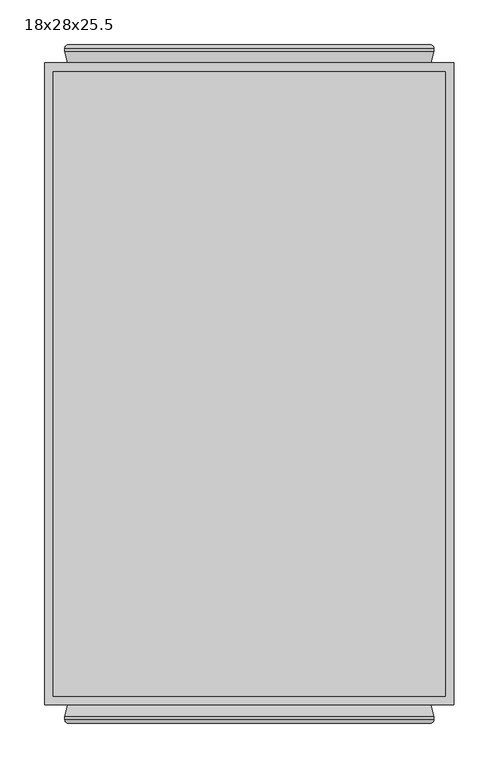
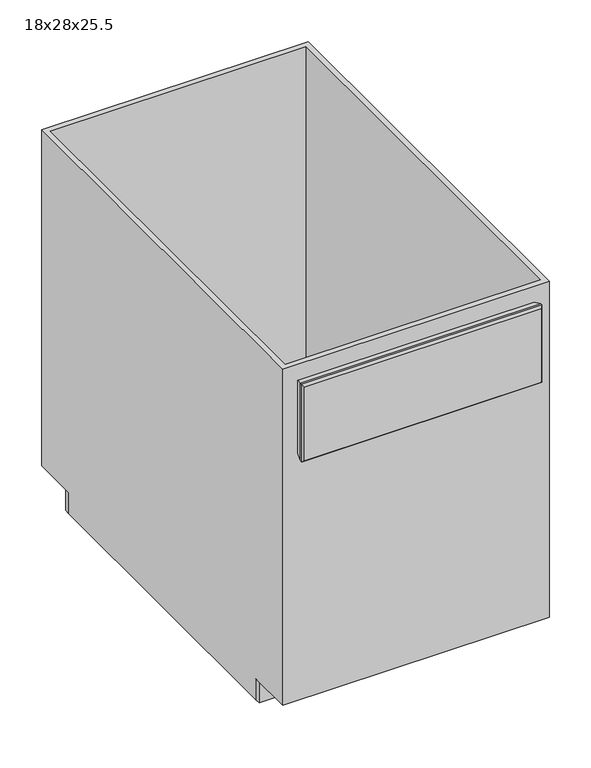
"""IFC4 building model written with IfcOpenShell, lengths in millimetres: furniture geometry, Cabinet-Base-Merillat-Peninsula_Single_Door-Marlin : 18x28x25.5."""

from ifc_helpers import new_model, si_unit, frame, origin, origin_with_axes, place, context, project, spatial, polyline, circle_curve, ellipse_curve, outline, extrude, faceted_brep, source, transform, mapped, element, save
from ifc_brep_helpers import plane_surface, cylinder_surface, advanced_brep


def furniture_18x28x25_5_8da4ed4e(model_context):
    return source(origin(), model_context, "Body", "SolidModel", [
        advanced_brep(
        [(225.1127049, 52.3621, 63.5), (222.0162124, 56.8325, 66.5964925), (222.0162124, 56.8325, 454.1035075), (225.1127049, 52.3621, 457.2), (225.1127049, 49.5935, 457.2), (225.1127049, 49.5935, 63.5), (221.6075049, 36.5125, 453.6948), (221.6075049, 36.5125, 67.0052), (176.9115422, 36.5125, 111.7011628), (176.9115422, 36.5125, 408.9988372), (176.5414105, 37.30625, 408.6287055), (174.4602514, 41.76931, 406.5475465), (174.4602514, 41.76931, 114.1524535), (176.5414105, 37.30625, 112.0712945), (175.8600209, 44.0094093, 407.947316), (175.8600209, 44.0094093, 112.752684), (190.1877049, 44.2595, 422.275), (190.1877049, 44.2595, 98.425), (190.1877049, 49.0855, 422.275), (190.1877049, 49.0855, 98.425), (175.8600209, 49.3355907, 407.947316), (175.8600209, 49.3355907, 112.752684), (174.4602514, 51.57569, 406.5475465), (174.4602514, 51.57569, 114.1524535), (176.5414105, 56.03875, 408.6287055), (176.9086747, 56.8263508, 408.9959698), (176.9115422, 56.8325, 111.7011628), (176.5414105, 56.03875, 112.0712945), (176.9086747, 56.8325, 454.1035075), (176.9086747, 52.3621, 457.2), (-184.5408026, 56.8325, 454.1035075), (-187.6372951, 52.3621, 457.2), (-139.4730764, 52.3621, 457.2), (-139.4730764, 56.8325, 454.1035075), (175.3211747, 52.3621, 457.2), (175.3211747, 56.8325, 454.1035075), (-137.8855764, 56.8325, 454.1035075), (-137.8855764, 52.3621, 457.2), (176.9086747, 49.5935, 457.2), (-187.6372951, 49.5935, 457.2), (-139.4730764, 49.5935, 457.2), (175.3211747, 49.5935, 457.2), (-137.8855764, 49.5935, 457.2), (176.9086747, 36.5125, 453.6948), (-184.1320951, 36.5125, 453.6948), (-139.4730764, 36.5125, 453.6948), (175.3211747, 36.5125, 453.6948), (-137.8855764, 36.5125, 453.6948), (-136.9848416, 41.76931, 406.5475465), (175.3211747, 37.30625, 408.6287055), (175.3211747, 36.5125, 408.9988372), (-137.8855764, 36.5125, 408.9988372), (-137.8855764, 37.30625, 408.6287055), (-139.0660006, 37.30625, 408.6287055), (-138.384611, 44.0094093, 407.947316), (-152.7122951, 44.2595, 422.275), (-152.7122951, 49.0855, 422.275), (-138.384611, 49.3355907, 407.947316), (-136.9848416, 51.57569, 406.5475465), (-139.0660006, 56.03875, 408.6287055), (-137.8855764, 56.03875, 408.6287055), (-137.8855764, 56.8325, 408.9988372), (175.3211747, 56.8325, 408.9988372), (175.3211747, 56.03875, 408.6287055), (-184.5408026, 56.8325, 66.5964925), (-187.6372951, 52.3621, 63.5), (-187.6372951, 49.5935, 63.5), (-184.1320951, 36.5125, 67.0052), (-139.4361323, 36.5125, 408.9988372), (-139.4361323, 36.5125, 111.7011628), (-139.0660006, 37.30625, 112.0712945), (-136.9848416, 41.76931, 114.1524535), (-138.384611, 44.0094093, 112.752684), (-152.7122951, 44.2595, 98.425), (-152.7122951, 49.0855, 98.425), (-138.384611, 49.3355907, 112.752684), (-136.9848416, 51.57569, 114.1524535), (-139.0660006, 56.03875, 112.0712945), (-139.4361323, 56.8325, 111.7011628), (-139.4361323, 56.8325, 408.9988372), (-139.4730764, 56.8325, 66.5964925), (-139.4730764, 52.3621, 63.5), (176.9086747, 52.3621, 63.5), (176.9086747, 56.8325, 66.5964925), (-137.8855764, 52.3621, 63.5), (-137.8855764, 56.8325, 66.5964925), (175.3211747, 56.8325, 66.5964925), (175.3211747, 52.3621, 63.5), (-139.4730764, 49.5935, 63.5), (176.9086747, 49.5935, 63.5), (-137.8855764, 49.5935, 63.5), (175.3211747, 49.5935, 63.5), (-139.4730764, 36.5125, 67.0052), (176.9086747, 36.5125, 67.0052), (-137.8855764, 36.5125, 67.0052), (175.3211747, 36.5125, 67.0052), (-137.8855764, 36.5125, 111.7011628), (175.3211747, 36.5125, 111.7011628), (-137.8855764, 37.30625, 112.0712945), (175.3211747, 37.30625, 112.0712945), (175.3211747, 56.03875, 112.0712945), (175.3211747, 56.8325, 111.7011628), (-137.8855764, 56.8325, 111.7011628), (-137.8855764, 56.03875, 112.0712945), (-137.8855764, 37.30625, 67.6142588), (-137.8855764, 49.6980037, 64.29375), (-137.8855764, 52.3621, 64.29375), (-137.8855764, 56.03875, 66.7473948), (-139.4730764, 56.03875, 112.0712945), (-139.4730764, 56.03875, 66.7473948), (-139.4730764, 52.3621, 64.29375), (-139.4730764, 49.6980037, 64.29375), (-139.4730764, 37.30625, 67.6142588), (-139.4730764, 37.30625, 112.0712945), (176.9086747, 37.30625, 112.0712945), (176.9086747, 37.30625, 67.6142588), (176.9086747, 49.6980037, 64.29375), (176.9086747, 52.3621, 64.29375), (176.9086747, 56.03875, 66.7473948), (176.9086747, 56.03875, 112.0712945), (175.3211747, 56.03875, 66.7473948), (175.3211747, 52.3621, 64.29375), (175.3211747, 49.6980037, 64.29375), (175.3211747, 37.30625, 67.6142588), (176.9086747, 56.03875, 408.6287055), (176.9086747, 56.03875, 453.9526052), (176.9086747, 52.3621, 456.40625), (176.9086747, 49.6980037, 456.40625), (176.9086747, 37.30625, 453.0857412), (176.9086747, 37.30625, 408.6287055), (175.3211747, 37.30625, 453.0857412), (175.3211747, 49.6980037, 456.40625), (175.3211747, 52.3621, 456.40625), (175.3211747, 56.03875, 453.9526052), (-137.8855764, 56.03875, 453.9526052), (-137.8855764, 52.3621, 456.40625), (-137.8855764, 49.6980037, 456.40625), (-137.8855764, 37.30625, 453.0857412), (-139.4730764, 56.03875, 408.6287055), (-139.4730764, 37.30625, 408.6287055), (-139.4730764, 37.30625, 453.0857412), (-139.4730764, 49.6980037, 456.40625), (-139.4730764, 52.3621, 456.40625), (-139.4730764, 56.03875, 453.9526052)],
        [
            (0, 1, ellipse_curve(frame((220.3375049, 52.3621, 68.2752), z_axis=(0.7071067811865498, 0.0, 0.7071067811865451), x_axis=(0.7071067811865451, 0.0, -0.70710678118655)), 6.7531526, 4.7752)),
            (1, 2),
            (2, 3, ellipse_curve(frame((220.3375049, 52.3621, 452.4248), z_axis=(0.7071067811865451, 0.0, -0.7071067811865498), x_axis=(-0.7071067811865497, 0.0, -0.7071067811865452)), 6.7531526, 4.7752)),
            (3, 0),
            (3, 4),
            (4, 5),
            (5, 0),
            (4, 6),
            (6, 7),
            (7, 5),
            (8, 9),
            (9, 10),
            (10, 11),
            (11, 12),
            (12, 13),
            (13, 8),
            (11, 14, ellipse_curve(frame((175.8875049, 42.4348492, 407.9748), z_axis=(0.7071067811865451, 0.0, -0.7071067811865498), x_axis=(-0.7071067811865497, 0.0, -0.7071067811865452)), 2.2271035, 1.5748)),
            (14, 15),
            (15, 12, ellipse_curve(frame((175.8875049, 42.4348492, 112.7252), z_axis=(0.7071067811865498, 0.0, 0.7071067811865451), x_axis=(0.7071067811865451, 0.0, -0.70710678118655)), 2.2271035, 1.5748)),
            (14, 16),
            (16, 17),
            (17, 15),
            (16, 18),
            (18, 19),
            (19, 17),
            (18, 20),
            (20, 21),
            (21, 19),
            (20, 22, ellipse_curve(frame((175.8875049, 50.9101508, 407.9748), z_axis=(0.7071067811865451, 0.0, -0.7071067811865498), x_axis=(-0.7071067811865497, 0.0, -0.7071067811865452)), 2.2271035, 1.5748)),
            (22, 23),
            (23, 21, ellipse_curve(frame((175.8875049, 50.9101508, 112.7252), z_axis=(0.7071067811865498, 0.0, 0.7071067811865451), x_axis=(0.7071067811865451, 0.0, -0.70710678118655)), 2.2271035, 1.5748)),
            (22, 24),
            (24, 25),
            (25, 26),
            (26, 27),
            (27, 23),
            (2, 28),
            (28, 29, circle_curve(frame((176.9086747, 52.3621, 452.4248), z_axis=(1.0, 0.0, 0.0), x_axis=(0.0, -1.0, 0.0)), 4.7752)),
            (29, 3),
            (30, 31, ellipse_curve(frame((-182.8620951, 52.3621, 452.4248), z_axis=(0.7071067811865498, 0.0, 0.7071067811865451), x_axis=(0.7071067811865452, 0.0, -0.7071067811865497)), 6.7531526, 4.7752)),
            (31, 32),
            (32, 33, circle_curve(frame((-139.4730764, 52.3621, 452.4248), z_axis=(-1.0, 0.0, 0.0), x_axis=(0.0, -1.0, 0.0)), 4.7752)),
            (33, 30),
            (34, 35, circle_curve(frame((175.3211747, 52.3621, 452.4248), z_axis=(-1.0, 0.0, 0.0), x_axis=(0.0, -1.0, 0.0)), 4.7752)),
            (35, 36),
            (36, 37, circle_curve(frame((-137.8855764, 52.3621, 452.4248), z_axis=(1.0, 0.0, 0.0), x_axis=(0.0, -1.0, 0.0)), 4.7752)),
            (37, 34),
            (29, 38),
            (38, 4),
            (31, 39),
            (39, 40),
            (40, 32),
            (41, 34),
            (37, 42),
            (42, 41),
            (38, 43),
            (43, 6),
            (39, 44),
            (44, 45),
            (45, 40),
            (46, 41),
            (42, 47),
            (47, 46),
            (48, 11),
            (10, 49),
            (49, 50),
            (50, 51),
            (51, 52),
            (52, 53),
            (53, 48),
            (48, 54, ellipse_curve(frame((-138.4120951, 42.4348492, 407.9748), z_axis=(0.7071067811865498, 0.0, 0.7071067811865451), x_axis=(0.7071067811865452, 0.0, -0.7071067811865497)), 2.2271035, 1.5748)),
            (54, 14),
            (54, 55),
            (55, 16),
            (55, 56),
            (56, 18),
            (56, 57),
            (57, 20),
            (57, 58, ellipse_curve(frame((-138.4120951, 50.9101508, 407.9748), z_axis=(0.7071067811865498, 0.0, 0.7071067811865451), x_axis=(0.7071067811865452, 0.0, -0.7071067811865497)), 2.2271035, 1.5748)),
            (58, 22),
            (58, 59),
            (59, 60),
            (60, 61),
            (61, 62),
            (62, 63),
            (63, 24),
            (30, 64),
            (64, 65, ellipse_curve(frame((-182.8620951, 52.3621, 68.2752), z_axis=(-0.7071067811865451, 0.0, 0.7071067811865498), x_axis=(0.7071067811865497, 0.0, 0.7071067811865452)), 6.7531526, 4.7752)),
            (65, 31),
            (65, 66),
            (66, 39),
            (66, 67),
            (67, 44),
            (68, 69),
            (69, 70),
            (70, 71),
            (71, 48),
            (53, 68),
            (71, 72, ellipse_curve(frame((-138.4120951, 42.4348492, 112.7252), z_axis=(-0.7071067811865451, 0.0, 0.7071067811865498), x_axis=(0.7071067811865497, 0.0, 0.7071067811865452)), 2.2271035, 1.5748)),
            (72, 54),
            (72, 73),
            (73, 55),
            (73, 74),
            (74, 56),
            (74, 75),
            (75, 57),
            (75, 76, ellipse_curve(frame((-138.4120951, 50.9101508, 112.7252), z_axis=(-0.7071067811865451, 0.0, 0.7071067811865498), x_axis=(0.7071067811865497, 0.0, 0.7071067811865452)), 2.2271035, 1.5748)),
            (76, 58),
            (76, 77),
            (77, 78),
            (78, 79),
            (79, 59),
            (64, 80),
            (80, 81, circle_curve(frame((-139.4730764, 52.3621, 68.2752), z_axis=(-1.0, 0.0, 0.0), x_axis=(0.0, -1.0, 0.0)), 4.7752)),
            (81, 65),
            (0, 82),
            (82, 83, circle_curve(frame((176.9086747, 52.3621, 68.2752), z_axis=(1.0, 0.0, 0.0), x_axis=(0.0, -1.0, 0.0)), 4.7752)),
            (83, 1),
            (84, 85, circle_curve(frame((-137.8855764, 52.3621, 68.2752), z_axis=(1.0, 0.0, 0.0), x_axis=(0.0, -1.0, 0.0)), 4.7752)),
            (85, 86),
            (86, 87, circle_curve(frame((175.3211747, 52.3621, 68.2752), z_axis=(-1.0, 0.0, 0.0), x_axis=(0.0, -1.0, 0.0)), 4.7752)),
            (87, 84),
            (81, 88),
            (88, 66),
            (5, 89),
            (89, 82),
            (90, 84),
            (87, 91),
            (91, 90),
            (88, 92),
            (92, 67),
            (7, 93),
            (93, 89),
            (94, 90),
            (91, 95),
            (95, 94),
            (43, 9),
            (8, 93),
            (92, 69),
            (68, 45),
            (96, 94),
            (95, 97),
            (97, 96),
            (50, 46),
            (47, 51),
            (12, 71),
            (70, 98),
            (98, 96),
            (97, 99),
            (99, 13),
            (15, 72),
            (17, 73),
            (19, 74),
            (21, 75),
            (23, 76),
            (27, 100),
            (100, 101),
            (101, 102),
            (102, 103),
            (103, 77),
            (83, 26),
            (25, 28),
            (33, 79),
            (78, 80),
            (85, 102),
            (101, 86),
            (35, 62),
            (61, 36),
            (98, 104),
            (104, 105),
            (105, 106),
            (106, 107, circle_curve(frame((-137.8855764, 52.3621, 68.2752), z_axis=(1.0, 0.0, 0.0), x_axis=(0.0, 0.0, -1.0)), 3.98145)),
            (107, 103),
            (78, 108),
            (108, 109),
            (109, 110, circle_curve(frame((-139.4730764, 52.3621, 68.2752), z_axis=(-1.0, 0.0, 0.0), x_axis=(0.0, 0.0, -1.0)), 3.98145)),
            (110, 111),
            (111, 112),
            (112, 113),
            (113, 69),
            (77, 108),
            (107, 109),
            (106, 110),
            (105, 111),
            (104, 112),
            (70, 113),
            (8, 114),
            (114, 115),
            (115, 116),
            (116, 117),
            (117, 118, circle_curve(frame((176.9086747, 52.3621, 68.2752), z_axis=(1.0, 0.0, 0.0), x_axis=(0.0, 0.0, -1.0)), 3.98145)),
            (118, 119),
            (119, 26),
            (100, 120),
            (120, 121, circle_curve(frame((175.3211747, 52.3621, 68.2752), z_axis=(-1.0, 0.0, 0.0), x_axis=(0.0, 0.0, -1.0)), 3.98145)),
            (121, 122),
            (122, 123),
            (123, 99),
            (119, 27),
            (118, 120),
            (117, 121),
            (116, 122),
            (115, 123),
            (114, 13),
            (25, 124),
            (124, 125),
            (125, 126, circle_curve(frame((176.9086747, 52.3621, 452.4248), z_axis=(1.0, 0.0, 0.0), x_axis=(0.0, 0.0, -1.0)), 3.98145)),
            (126, 127),
            (127, 128),
            (128, 129),
            (129, 9),
            (49, 130),
            (130, 131),
            (131, 132),
            (132, 133, circle_curve(frame((175.3211747, 52.3621, 452.4248), z_axis=(-1.0, 0.0, 0.0), x_axis=(0.0, 0.0, -1.0)), 3.98145)),
            (133, 63),
            (129, 10),
            (128, 130),
            (127, 131),
            (126, 132),
            (125, 133),
            (124, 24),
            (60, 134),
            (134, 135, circle_curve(frame((-137.8855764, 52.3621, 452.4248), z_axis=(1.0, 0.0, 0.0), x_axis=(0.0, 0.0, -1.0)), 3.98145)),
            (135, 136),
            (136, 137),
            (137, 52),
            (138, 79),
            (68, 139),
            (139, 140),
            (140, 141),
            (141, 142),
            (142, 143, circle_curve(frame((-139.4730764, 52.3621, 452.4248), z_axis=(-1.0, 0.0, 0.0), x_axis=(0.0, 0.0, -1.0)), 3.98145)),
            (143, 138),
            (138, 59),
            (53, 139),
            (137, 140),
            (136, 141),
            (135, 142),
            (134, 143),
        ],
        [
            cylinder_surface(frame((220.3375049, 52.3621, 63.5), z_axis=(0.0, 0.0, -1.0), x_axis=(0.0, -1.0, 0.0)), 4.7752),
            plane_surface(frame((225.1127049, 52.3621, 63.5), z_axis=(1.0, 0.0, 0.0), x_axis=(0.0, 0.0, 1.0))),
            plane_surface(frame((225.1127049, 49.5935, 63.5), z_axis=(0.9659229350723619, -0.25882983502910506, 0.0), x_axis=(0.0, 0.0, 1.0))),
            plane_surface(frame((176.9115422, 36.5125, 111.7011628), z_axis=(-0.9063077870366099, -0.4226182617407856, 0.0), x_axis=(0.0, 0.0, 1.0))),
            cylinder_surface(frame((175.8875049, 42.4348492, 63.5), z_axis=(0.0, 0.0, -1.0000000000000002), x_axis=(-0.01745240643729364, 0.9998476951563912, 0.0)), 1.5748),
            plane_surface(frame((175.8600209, 44.0094093, 112.752684), z_axis=(-0.017452406437322144, 0.9998476951563906, 0.0), x_axis=(0.0, 0.0, 1.0))),
            plane_surface(frame((190.1877049, 44.2595, 98.425), z_axis=(-1.0, 0.0, 0.0), x_axis=(0.0, 0.0, 1.0))),
            plane_surface(frame((190.1877049, 49.0855, 98.425), z_axis=(-0.01745240643727848, -0.9998476951563914, 0.0), x_axis=(0.0, 0.0, 1.0))),
            cylinder_surface(frame((175.8875049, 50.9101508, 63.5), z_axis=(0.0, 0.0, -1.0000000000000002), x_axis=(-0.9063077870367326, 0.42261826174052236, 0.0)), 1.5748),
            plane_surface(frame((174.4602514, 51.57569, 114.1524535), z_axis=(-0.9063077870366333, 0.4226182617407352, 0.0), x_axis=(0.0, 0.0, 1.0))),
            cylinder_surface(frame((225.1127049, 52.3621, 452.4248), z_axis=(1.0, 0.0, 0.0), x_axis=(0.0, -1.0, 0.0)), 4.7752),
            plane_surface(frame((225.1127049, 52.3621, 457.2), z_axis=(0.0, 0.0, 1.0), x_axis=(-1.0, 0.0, 0.0))),
            plane_surface(frame((225.1127049, 49.5935, 457.2), z_axis=(0.0, -0.25882983502910506, 0.9659229350723619), x_axis=(-1.0, 0.0, 0.0))),
            plane_surface(frame((176.9115422, 36.5125, 408.9988372), z_axis=(0.0, -0.4226182617407856, -0.9063077870366099), x_axis=(-1.0, 0.0, 0.0))),
            cylinder_surface(frame((225.1127049, 42.4348492, 407.9748), z_axis=(1.0000000000000002, 0.0, 0.0), x_axis=(0.0, 0.9998476951563912, -0.01745240643729364)), 1.5748),
            plane_surface(frame((175.8600209, 44.0094093, 407.947316), z_axis=(0.0, 0.9998476951563906, -0.017452406437322144), x_axis=(-1.0, 0.0, 0.0))),
            plane_surface(frame((190.1877049, 44.2595, 422.275), z_axis=(0.0, 0.0, -1.0), x_axis=(-1.0, 0.0, 0.0))),
            plane_surface(frame((190.1877049, 49.0855, 422.275), z_axis=(0.0, -0.9998476951563914, -0.01745240643727848), x_axis=(-1.0, 0.0, 0.0))),
            cylinder_surface(frame((225.1127049, 50.9101508, 407.9748), z_axis=(1.0000000000000002, 0.0, 0.0), x_axis=(0.0, 0.42261826174052236, -0.9063077870367326)), 1.5748),
            plane_surface(frame((174.4602514, 51.57569, 406.5475465), z_axis=(0.0, 0.4226182617407352, -0.9063077870366333), x_axis=(-1.0, 0.0, 0.0))),
            cylinder_surface(frame((-182.8620951, 52.3621, 457.2), z_axis=(0.0, 0.0, 1.0), x_axis=(0.0, -1.0, 0.0)), 4.7752),
            plane_surface(frame((-187.6372951, 52.3621, 457.2), z_axis=(-1.0, 0.0, 0.0), x_axis=(0.0, 0.0, -1.0))),
            plane_surface(frame((-187.6372951, 49.5935, 457.2), z_axis=(-0.9659229350723619, -0.25882983502910506, 0.0), x_axis=(0.0, 0.0, -1.0))),
            plane_surface(frame((-139.4361323, 36.5125, 408.9988372), z_axis=(0.9063077870366099, -0.4226182617407856, 0.0), x_axis=(0.0, 0.0, -1.0))),
            cylinder_surface(frame((-138.4120951, 42.4348492, 457.2), z_axis=(0.0, 0.0, 1.0000000000000002), x_axis=(0.01745240643729364, 0.9998476951563912, 0.0)), 1.5748),
            plane_surface(frame((-138.384611, 44.0094093, 407.947316), z_axis=(0.017452406437322144, 0.9998476951563906, 0.0), x_axis=(0.0, 0.0, -1.0))),
            plane_surface(frame((-152.7122951, 44.2595, 422.275), z_axis=(1.0, 0.0, 0.0), x_axis=(0.0, 0.0, -1.0))),
            plane_surface(frame((-152.7122951, 49.0855, 422.275), z_axis=(0.01745240643727848, -0.9998476951563914, 0.0), x_axis=(0.0, 0.0, -1.0))),
            cylinder_surface(frame((-138.4120951, 50.9101508, 457.2), z_axis=(0.0, 0.0, 1.0000000000000002), x_axis=(0.9063077870367326, 0.42261826174052236, 0.0)), 1.5748),
            plane_surface(frame((-136.9848416, 51.57569, 406.5475465), z_axis=(0.9063077870366333, 0.4226182617407352, 0.0), x_axis=(0.0, 0.0, -1.0))),
            cylinder_surface(frame((-187.6372951, 52.3621, 68.2752), z_axis=(-1.0, 0.0, 0.0), x_axis=(0.0, -1.0, 0.0)), 4.7752),
            plane_surface(frame((-187.6372951, 52.3621, 63.5), z_axis=(0.0, 0.0, -1.0), x_axis=(1.0, 0.0, 0.0))),
            plane_surface(frame((-187.6372951, 49.5935, 63.5), z_axis=(0.0, -0.25882983502910506, -0.9659229350723619), x_axis=(1.0, 0.0, 0.0))),
            plane_surface(frame((-184.1320951, 36.5125, 67.0052), z_axis=(0.0, -1.0, 0.0), x_axis=(1.0, 0.0, 0.0))),
            plane_surface(frame((-139.4361323, 36.5125, 111.7011628), z_axis=(0.0, -0.4226182617407856, 0.9063077870366099), x_axis=(1.0, 0.0, 0.0))),
            cylinder_surface(frame((-187.6372951, 42.4348492, 112.7252), z_axis=(-1.0000000000000002, 0.0, 0.0), x_axis=(0.0, 0.9998476951563912, 0.01745240643729364)), 1.5748),
            plane_surface(frame((-138.384611, 44.0094093, 112.752684), z_axis=(0.0, 0.9998476951563906, 0.017452406437322144), x_axis=(1.0, 0.0, 0.0))),
            plane_surface(frame((-152.7122951, 44.2595, 98.425), z_axis=(0.0, 0.0, 1.0), x_axis=(1.0, 0.0, 0.0))),
            plane_surface(frame((-152.7122951, 49.0855, 98.425), z_axis=(0.0, -0.9998476951563914, 0.01745240643727848), x_axis=(1.0, 0.0, 0.0))),
            cylinder_surface(frame((-187.6372951, 50.9101508, 112.7252), z_axis=(-1.0000000000000002, 0.0, 0.0), x_axis=(0.0, 0.42261826174052236, 0.9063077870367326)), 1.5748),
            plane_surface(frame((-136.9848416, 51.57569, 114.1524535), z_axis=(0.0, 0.4226182617407352, 0.9063077870366333), x_axis=(1.0, 0.0, 0.0))),
            plane_surface(frame((-139.4361323, 56.8325, 111.7011628), z_axis=(0.0, 1.0, 0.0), x_axis=(1.0, 0.0, 0.0))),
            plane_surface(frame((-137.8855764, 56.8325, 111.7011628), z_axis=(-1.0000000000000002, 0.0, 0.0), x_axis=(0.0, -0.9063077870366303, 0.4226182617407418))),
            plane_surface(frame((-139.4730764, 56.8325, 111.7011628), z_axis=(1.0000000000000002, 0.0, 0.0), x_axis=(0.0, 0.9063077870366303, -0.4226182617407418))),
            plane_surface(frame((-137.8855764, 56.8325, 111.7011628), z_axis=(0.0, -0.4226182617407418, -0.9063077870366303), x_axis=(-1.0, 0.0, 0.0))),
            plane_surface(frame((-137.8855764, 56.03875, 112.0712945), z_axis=(0.0, 1.0, 0.0), x_axis=(-1.0, 0.0, 0.0))),
            cylinder_surface(frame((-139.4730764, 52.3621, 68.2752), z_axis=(-1.0, 0.0, 0.0), x_axis=(0.0, 0.0, -1.0)), 3.98145),
            plane_surface(frame((-137.8855764, 52.3621, 64.29375), z_axis=(0.0, 0.0, -1.0), x_axis=(-1.0, 0.0, 0.0))),
            plane_surface(frame((-137.8855764, 49.6980037, 64.29375), z_axis=(0.0, -0.25882983502916795, -0.9659229350723451), x_axis=(-1.0, 0.0, 0.0))),
            plane_surface(frame((-137.8855764, 37.30625, 67.6142588), z_axis=(0.0, -1.0, 0.0), x_axis=(-1.0, 0.0, 0.0))),
            plane_surface(frame((-137.8855764, 37.30625, 112.0712945), z_axis=(0.0, 0.4226182617407951, -0.9063077870366054), x_axis=(-1.0, 0.0, 0.0))),
            plane_surface(frame((176.9086747, 56.8325, 111.7011628), z_axis=(-1.0, 0.0, 0.0), x_axis=(0.0, -0.9063077870366284, 0.42261826174074574))),
            plane_surface(frame((175.3211747, 56.8325, 111.7011628), z_axis=(1.0, 0.0, 0.0), x_axis=(0.0, 0.9063077870366284, -0.42261826174074574))),
            plane_surface(frame((176.9086747, 56.8325, 111.7011628), z_axis=(0.0, -0.42261826174074574, -0.9063077870366284), x_axis=(-1.0, 0.0, 0.0))),
            plane_surface(frame((176.9086747, 56.03875, 112.0712945), z_axis=(0.0, 1.0, 0.0), x_axis=(-1.0, 0.0, 0.0))),
            cylinder_surface(frame((175.3211747, 52.3621, 68.2752), z_axis=(-1.0, 0.0, 0.0), x_axis=(0.0, 0.0, -1.0)), 3.98145),
            plane_surface(frame((176.9086747, 52.3621, 64.29375), z_axis=(0.0, 0.0, -1.0), x_axis=(-1.0, 0.0, 0.0))),
            plane_surface(frame((176.9086747, 49.6980037, 64.29375), z_axis=(0.0, -0.25882983502917023, -0.9659229350723445), x_axis=(-1.0, 0.0, 0.0))),
            plane_surface(frame((176.9086747, 37.30625, 67.6142588), z_axis=(0.0, -1.0, 0.0), x_axis=(-1.0, 0.0, 0.0))),
            plane_surface(frame((176.9086747, 37.30625, 112.0712945), z_axis=(0.0, 0.4226182617408056, -0.9063077870366005), x_axis=(-1.0, 0.0, 0.0))),
            plane_surface(frame((176.9086747, 52.3621, 447.6496), z_axis=(-1.0, 0.0, 0.0), x_axis=(0.0, 1.0, 0.0))),
            plane_surface(frame((175.3211747, 52.3621, 447.6496), z_axis=(1.0, 0.0, 0.0), x_axis=(0.0, -1.0, 0.0))),
            plane_surface(frame((176.9086747, 36.5125, 408.9988372), z_axis=(0.0, 0.4226182617407918, 0.906307787036607), x_axis=(-1.0, 0.0, 0.0))),
            plane_surface(frame((176.9086747, 37.30625, 408.6287055), z_axis=(0.0, -1.0, 0.0), x_axis=(-1.0, 0.0, 0.0))),
            plane_surface(frame((176.9086747, 37.30625, 453.0857412), z_axis=(0.0, -0.25882983502943885, 0.9659229350722724), x_axis=(-1.0, 0.0, 0.0))),
            plane_surface(frame((176.9086747, 49.6980037, 456.40625), z_axis=(0.0, 0.0, 1.0), x_axis=(-1.0, 0.0, 0.0))),
            cylinder_surface(frame((175.3211747, 52.3621, 452.4248), z_axis=(-1.0, 0.0, 0.0), x_axis=(0.0, 0.0, -1.0)), 3.98145),
            plane_surface(frame((176.9086747, 56.03875, 453.9526052), z_axis=(0.0, 1.0, 0.0), x_axis=(-1.0, 0.0, 0.0))),
            plane_surface(frame((176.9086747, 56.03875, 408.6287055), z_axis=(0.0, -0.42261826174073464, 0.9063077870366336), x_axis=(-1.0, 0.0, 0.0))),
            plane_surface(frame((-137.8855764, 56.03875, 408.6287055), z_axis=(-1.0, 0.0, 0.0), x_axis=(0.0, 0.9063077870366311, 0.4226182617407399))),
            plane_surface(frame((-139.4730764, 56.03875, 408.6287055), z_axis=(1.0, 0.0, 0.0), x_axis=(0.0, -0.9063077870366311, -0.4226182617407399))),
            plane_surface(frame((-137.8855764, 56.03875, 408.6287055), z_axis=(0.0, -0.4226182617407399, 0.9063077870366311), x_axis=(-1.0, 0.0, 0.0))),
            plane_surface(frame((-137.8855764, 36.5125, 408.9988372), z_axis=(0.0, 0.42261826174079353, 0.9063077870366061), x_axis=(-1.0, 0.0, 0.0))),
            plane_surface(frame((-137.8855764, 37.30625, 408.6287055), z_axis=(0.0, -1.0, 0.0), x_axis=(-1.0, 0.0, 0.0))),
            plane_surface(frame((-137.8855764, 37.30625, 453.0857412), z_axis=(0.0, -0.2588298350294384, 0.9659229350722726), x_axis=(-1.0, 0.0, 0.0))),
            plane_surface(frame((-137.8855764, 49.6980037, 456.40625), z_axis=(0.0, 0.0, 1.0), x_axis=(-1.0, 0.0, 0.0))),
            cylinder_surface(frame((-139.4730764, 52.3621, 452.4248), z_axis=(-1.0, 0.0, 0.0), x_axis=(0.0, 0.0, -1.0)), 3.98145),
            plane_surface(frame((-137.8855764, 56.03875, 453.9526052), z_axis=(0.0, 1.0, 0.0), x_axis=(-1.0, 0.0, 0.0))),
        ],
        [
            (0, [[1, 2, 3, 4]]),
            (1, [[-4, 5, 6, 7]]),
            (2, [[-6, 8, 9, 10]]),
            (3, [[11, 12, 13, 14, 15, 16]]),
            (4, [[-14, 17, 18, 19]]),
            (5, [[-18, 20, 21, 22]]),
            (6, [[-21, 23, 24, 25]]),
            (7, [[-24, 26, 27, 28]]),
            (8, [[-27, 29, 30, 31]]),
            (9, [[-30, 32, 33, 34, 35, 36]]),
            (10, [[-3, 37, 38, 39]]),
            (10, [[40, 41, 42, 43]]),
            (10, [[44, 45, 46, 47]]),
            (11, [[-5, -39, 48, 49]]),
            (11, [[50, 51, 52, -41]]),
            (11, [[53, -47, 54, 55]]),
            (12, [[-8, -49, 56, 57]]),
            (12, [[58, 59, 60, -51]]),
            (12, [[61, -55, 62, 63]]),
            (13, [[64, -13, 65, 66, 67, 68, 69, 70]]),
            (14, [[-17, -64, 71, 72]]),
            (15, [[-20, -72, 73, 74]]),
            (16, [[-23, -74, 75, 76]]),
            (17, [[-26, -76, 77, 78]]),
            (18, [[-29, -78, 79, 80]]),
            (19, [[-80, 81, 82, 83, 84, 85, 86, -32]]),
            (20, [[-40, 87, 88, 89]]),
            (21, [[-50, -89, 90, 91]]),
            (22, [[-58, -91, 92, 93]]),
            (23, [[94, 95, 96, 97, -70, 98]]),
            (24, [[-71, -97, 99, 100]]),
            (25, [[-73, -100, 101, 102]]),
            (26, [[-75, -102, 103, 104]]),
            (27, [[-77, -104, 105, 106]]),
            (28, [[-79, -106, 107, 108]]),
            (29, [[-108, 109, 110, 111, 112, -81]]),
            (30, [[-88, 113, 114, 115]]),
            (30, [[-1, 116, 117, 118]]),
            (30, [[119, 120, 121, 122]]),
            (31, [[-90, -115, 123, 124]]),
            (31, [[-7, 125, 126, -116]]),
            (31, [[127, -122, 128, 129]]),
            (32, [[-92, -124, 130, 131]]),
            (32, [[-10, 132, 133, -125]]),
            (32, [[134, -129, 135, 136]]),
            (33, [[-9, -57, 137, -11, 138, -132]]),
            (33, [[-93, -131, 139, -94, 140, -59]]),
            (33, [[141, -136, 142, 143]]),
            (33, [[144, -63, 145, -67]]),
            (34, [[146, -96, 147, 148, -143, 149, 150, -15]]),
            (35, [[-19, 151, -99, -146]]),
            (36, [[-22, 152, -101, -151]]),
            (37, [[-25, 153, -103, -152]]),
            (38, [[-28, 154, -105, -153]]),
            (39, [[-31, 155, -107, -154]]),
            (40, [[-155, -36, 156, 157, 158, 159, 160, -109]]),
            (41, [[-2, -118, 161, -34, 162, -37]]),
            (41, [[-87, -43, 163, -111, 164, -113]]),
            (41, [[165, -158, 166, -120]]),
            (41, [[167, -84, 168, -45]]),
            (42, [[169, 170, 171, 172, 173, -159, -165, -119, -127, -134, -141, -148]]),
            (43, [[174, 175, 176, 177, 178, 179, 180, -139, -130, -123, -114, -164]]),
            (44, [[-174, -110, 181]]),
            (45, [[-173, 182, -175, -181, -160]]),
            (46, [[-172, 183, -176, -182]]),
            (47, [[-171, 184, -177, -183]]),
            (48, [[-170, 185, -178, -184]]),
            (49, [[-169, -147, 186, -179, -185]]),
            (50, [[-180, -186, -95]]),
            (51, [[187, 188, 189, 190, 191, 192, 193, -161, -117, -126, -133, -138]]),
            (52, [[194, 195, 196, 197, 198, -149, -142, -135, -128, -121, -166, -157]]),
            (53, [[-193, 199, -35]]),
            (54, [[-192, 200, -194, -156, -199]]),
            (55, [[-191, 201, -195, -200]]),
            (56, [[-190, 202, -196, -201]]),
            (57, [[-189, 203, -197, -202]]),
            (58, [[-188, 204, -150, -198, -203]]),
            (59, [[-187, -16, -204]]),
            (60, [[205, 206, 207, 208, 209, 210, 211, -137, -56, -48, -38, -162]]),
            (61, [[212, 213, 214, 215, 216, -85, -167, -44, -53, -61, -144, -66]]),
            (62, [[-211, 217, -12]]),
            (63, [[-210, 218, -212, -65, -217]]),
            (64, [[-209, 219, -213, -218]]),
            (65, [[-208, 220, -214, -219]]),
            (66, [[-207, 221, -215, -220]]),
            (67, [[-206, 222, -86, -216, -221]]),
            (68, [[-205, -33, -222]]),
            (69, [[223, 224, 225, 226, 227, -68, -145, -62, -54, -46, -168, -83]]),
            (70, [[228, -163, -42, -52, -60, -140, 229, 230, 231, 232, 233, 234]]),
            (71, [[-228, 235, -112]]),
            (72, [[-229, -98, 236]]),
            (73, [[-227, 237, -230, -236, -69]]),
            (74, [[-226, 238, -231, -237]]),
            (75, [[-225, 239, -232, -238]]),
            (76, [[-224, 240, -233, -239]]),
            (77, [[-223, -82, -235, -234, -240]]),
        ],
    ),
        extrude(outline(polyline([(-152.7122951, 49.0855), (190.1877049, 49.0855), (190.1877049, 44.2595), (-152.7122951, 44.2595), (-152.7122951, 49.0855)])), frame((0.0, 0.0, 98.425), z_axis=(0.0, 0.0, 1.0), x_axis=(1.0, 0.0, 0.0)), (0.0, 0.0, 1.0), 323.85),
        advanced_brep(
        [(222.0162124, 56.8325, 619.2035075), (222.0162124, 56.8325, 485.6964925), (-184.5408026, 56.8325, 485.6964925), (-184.5408026, 56.8325, 619.2035075), (221.6075049, 36.5125, 486.1052), (221.6075049, 36.5125, 618.7948), (-184.1320951, 36.5125, 618.7948), (-184.1320951, 36.5125, 486.1052), (225.1127049, 52.3621, 622.3), (225.1127049, 49.5935, 622.3), (225.1127049, 49.5935, 482.6), (225.1127049, 52.3621, 482.6), (-187.6372951, 49.5935, 482.6), (-187.6372951, 52.3621, 482.6), (-187.6372951, 49.5935, 622.3), (-187.6372951, 52.3621, 622.3)],
        [
            (0, 1),
            (1, 2),
            (2, 3),
            (3, 0),
            (4, 5),
            (5, 6),
            (6, 7),
            (7, 4),
            (8, 9),
            (9, 10),
            (10, 11),
            (11, 8),
            (10, 12),
            (12, 13),
            (13, 11),
            (12, 14),
            (14, 15),
            (15, 13),
            (8, 15),
            (14, 9),
            (11, 1, ellipse_curve(frame((220.3375049, 52.3621, 487.3752), z_axis=(0.7071067811865498, 0.0, 0.7071067811865451), x_axis=(0.7071067811865451, 0.0, -0.70710678118655)), 6.7531526, 4.7752)),
            (0, 8, ellipse_curve(frame((220.3375049, 52.3621, 617.5248), z_axis=(0.7071067811865451, 0.0, -0.7071067811865498), x_axis=(-0.7071067811865497, 0.0, -0.7071067811865452)), 6.7531526, 4.7752)),
            (4, 10),
            (9, 5),
            (13, 2, ellipse_curve(frame((-182.8620951, 52.3621, 487.3752), z_axis=(0.7071067811865451, 0.0, -0.7071067811865498), x_axis=(-0.70710678118655, 0.0, -0.7071067811865451)), 6.7531526, 4.7752)),
            (7, 12),
            (15, 3, ellipse_curve(frame((-182.8620951, 52.3621, 617.5248), z_axis=(-0.7071067811865498, 0.0, -0.7071067811865451), x_axis=(-0.7071067811865451, 0.0, 0.70710678118655)), 6.7531526, 4.7752)),
            (6, 14),
        ],
        [
            plane_surface(frame((225.1127049, 56.8325, 622.3), z_axis=(0.0, 1.0, 0.0), x_axis=(0.0, 0.0, -1.0))),
            plane_surface(frame((225.1127049, 36.5125, 622.3), z_axis=(0.0, -1.0, 0.0), x_axis=(0.0, 0.0, 1.0))),
            plane_surface(frame((225.1127049, 56.8325, 622.3), z_axis=(1.0, 0.0, 0.0), x_axis=(0.0, -1.0, 0.0))),
            plane_surface(frame((225.1127049, 56.8325, 482.6), z_axis=(0.0, 0.0, -1.0), x_axis=(0.0, -1.0, 0.0))),
            plane_surface(frame((-187.6372951, 56.8325, 482.6), z_axis=(-1.0, 0.0, 0.0), x_axis=(0.0, -1.0, 0.0))),
            plane_surface(frame((-187.6372951, 56.8325, 622.3), z_axis=(0.0, 0.0, 1.0), x_axis=(0.0, -1.0, 0.0))),
            cylinder_surface(frame((220.3375049, 52.3621, 622.3), z_axis=(0.0, 0.0, -1.0), x_axis=(0.0, -1.0, 0.0)), 4.7752),
            plane_surface(frame((225.1127049, 49.5935, 622.3), z_axis=(0.9659229350723619, -0.25882983502910506, 0.0), x_axis=(0.0, 0.0, -1.0))),
            cylinder_surface(frame((225.1127049, 52.3621, 487.3752), z_axis=(-1.0, 0.0, 0.0), x_axis=(0.0, -1.0, 0.0)), 4.7752),
            plane_surface(frame((225.1127049, 49.5935, 482.6), z_axis=(0.0, -0.25882983502910506, -0.9659229350723619), x_axis=(-1.0, 0.0, 0.0))),
            cylinder_surface(frame((-182.8620951, 52.3621, 482.6), z_axis=(0.0, 0.0, 1.0), x_axis=(0.0, -1.0, 0.0)), 4.7752),
            plane_surface(frame((-187.6372951, 49.5935, 482.6), z_axis=(-0.9659229350723619, -0.25882983502910506, 0.0), x_axis=(0.0, 0.0, 1.0))),
            cylinder_surface(frame((-187.6372951, 52.3621, 617.5248), z_axis=(1.0, 0.0, 0.0), x_axis=(0.0, -1.0, 0.0)), 4.7752),
            plane_surface(frame((-187.6372951, 49.5935, 622.3), z_axis=(0.0, -0.25882983502910506, 0.9659229350723619), x_axis=(1.0, 0.0, 0.0))),
        ],
        [
            (0, [[1, 2, 3, 4]]),
            (1, [[5, 6, 7, 8]]),
            (2, [[9, 10, 11, 12]]),
            (3, [[-11, 13, 14, 15]]),
            (4, [[-14, 16, 17, 18]]),
            (5, [[-9, 19, -17, 20]]),
            (6, [[21, -1, 22, -12]]),
            (7, [[23, -10, 24, -5]]),
            (8, [[-21, -15, 25, -2]]),
            (9, [[-23, -8, 26, -13]]),
            (10, [[-25, -18, 27, -3]]),
            (11, [[-26, -7, 28, -16]]),
            (12, [[-22, -4, -27, -19]]),
            (13, [[-24, -20, -28, -6]]),
        ],
    ),
        advanced_brep(
        [(-184.5408026, -700.56375, 619.2035075), (-184.5408026, -700.56375, 485.6964925), (222.0162124, -700.56375, 485.6964925), (222.0162124, -700.56375, 619.2035075), (-184.1320951, -680.24375, 486.1052), (-184.1320951, -680.24375, 618.7948), (221.6075049, -680.24375, 618.7948), (221.6075049, -680.24375, 486.1052), (-187.6372951, -696.09335, 622.3), (-187.6372951, -693.32475, 622.3), (-187.6372951, -693.32475, 482.6), (-187.6372951, -696.09335, 482.6), (225.1127049, -693.32475, 482.6), (225.1127049, -696.09335, 482.6), (225.1127049, -693.32475, 622.3), (225.1127049, -696.09335, 622.3)],
        [
            (0, 1),
            (1, 2),
            (2, 3),
            (3, 0),
            (4, 5),
            (5, 6),
            (6, 7),
            (7, 4),
            (8, 9),
            (9, 10),
            (10, 11),
            (11, 8),
            (10, 12),
            (12, 13),
            (13, 11),
            (12, 14),
            (14, 15),
            (15, 13),
            (8, 15),
            (14, 9),
            (11, 1, ellipse_curve(frame((-182.8620951, -696.09335, 487.3752), z_axis=(-0.7071067811865475, 0.0, 0.7071067811865475), x_axis=(-0.7071067811865474, 0.0, -0.7071067811865476)), 6.7531526, 4.7752)),
            (0, 8, ellipse_curve(frame((-182.8620951, -696.09335, 617.5248), z_axis=(-0.7071067811865475, 0.0, -0.7071067811865475), x_axis=(0.7071067811865474, 0.0, -0.7071067811865476)), 6.7531526, 4.7752)),
            (4, 10),
            (9, 5),
            (13, 2, ellipse_curve(frame((220.3375049, -696.09335, 487.3752), z_axis=(-0.7071067811865475, 0.0, -0.7071067811865475), x_axis=(0.7071067811865476, 0.0, -0.7071067811865474)), 6.7531526, 4.7752)),
            (7, 12),
            (15, 3, ellipse_curve(frame((220.3375049, -696.09335, 617.5248), z_axis=(0.7071067811865475, 0.0, -0.7071067811865475), x_axis=(0.7071067811865474, 0.0, 0.7071067811865476)), 6.7531526, 4.7752)),
            (6, 14),
        ],
        [
            plane_surface(frame((-187.6372951, -700.56375, 622.3), z_axis=(0.0, -1.0, 0.0), x_axis=(0.0, 0.0, -1.0))),
            plane_surface(frame((-187.6372951, -680.24375, 622.3), z_axis=(0.0, 1.0, 0.0), x_axis=(0.0, 0.0, 1.0))),
            plane_surface(frame((-187.6372951, -700.56375, 622.3), z_axis=(-1.0, 0.0, 0.0), x_axis=(0.0, 1.0, 0.0))),
            plane_surface(frame((-187.6372951, -700.56375, 482.6), z_axis=(0.0, 0.0, -1.0), x_axis=(0.0, 1.0, 0.0))),
            plane_surface(frame((225.1127049, -700.56375, 482.6), z_axis=(1.0, 0.0, 0.0), x_axis=(0.0, 1.0, 0.0))),
            plane_surface(frame((225.1127049, -700.56375, 622.3), z_axis=(0.0, 0.0, 1.0), x_axis=(0.0, 1.0, 0.0))),
            cylinder_surface(frame((-182.8620951, -696.09335, 622.3), z_axis=(0.0, 0.0, -1.0), x_axis=(0.0, 1.0, 0.0)), 4.7752),
            plane_surface(frame((-187.6372951, -693.32475, 622.3), z_axis=(-0.9659229350723619, 0.25882983502910506, 0.0), x_axis=(0.0, 0.0, -1.0))),
            cylinder_surface(frame((-187.6372951, -696.09335, 487.3752), z_axis=(1.0, 0.0, 0.0), x_axis=(0.0, 1.0, 0.0)), 4.7752),
            plane_surface(frame((-187.6372951, -693.32475, 482.6), z_axis=(0.0, 0.25882983502910506, -0.9659229350723619), x_axis=(1.0, 0.0, 0.0))),
            cylinder_surface(frame((220.3375049, -696.09335, 482.6), z_axis=(0.0, 0.0, 1.0), x_axis=(0.0, 1.0, 0.0)), 4.7752),
            plane_surface(frame((225.1127049, -693.32475, 482.6), z_axis=(0.9659229350723619, 0.25882983502910506, 0.0), x_axis=(0.0, 0.0, 1.0))),
            cylinder_surface(frame((225.1127049, -696.09335, 617.5248), z_axis=(-1.0, 0.0, 0.0), x_axis=(0.0, 1.0, 0.0)), 4.7752),
            plane_surface(frame((225.1127049, -693.32475, 622.3), z_axis=(0.0, 0.25882983502910506, 0.9659229350723619), x_axis=(-1.0, 0.0, 0.0))),
        ],
        [
            (0, [[1, 2, 3, 4]]),
            (1, [[5, 6, 7, 8]]),
            (2, [[9, 10, 11, 12]]),
            (3, [[-11, 13, 14, 15]]),
            (4, [[-14, 16, 17, 18]]),
            (5, [[-9, 19, -17, 20]]),
            (6, [[21, -1, 22, -12]]),
            (7, [[23, -10, 24, -5]]),
            (8, [[-21, -15, 25, -2]]),
            (9, [[-23, -8, 26, -13]]),
            (10, [[-25, -18, 27, -3]]),
            (11, [[-26, -7, 28, -16]]),
            (12, [[-22, -4, -27, -19]]),
            (13, [[-24, -20, -28, -6]]),
        ],
    ),
        faceted_brep([(247.3377049, 36.5125, 647.7), (-209.8622951, 36.5125, 647.7), (-209.8622951, -680.24375, 647.7), (247.3377049, -680.24375, 647.7), (237.8127049, 26.9875, 647.7), (237.8127049, -670.71875, 647.7), (-200.3372951, -670.71875, 647.7), (-200.3372951, 26.9875, 647.7), (247.3377049, -680.24375, 38.1), (-209.8622951, -680.24375, 38.1), (-209.8622951, -600.075, 38.1), (-200.3372951, -600.075, 38.1), (-200.3372951, -43.65625, 38.1), (-209.8622951, -43.65625, 38.1), (-209.8622951, 36.5125, 38.1), (247.3377049, 36.5125, 38.1), (247.3377049, -43.65625, 38.1), (237.8127049, -43.65625, 38.1), (237.8127049, -600.075, 38.1), (247.3377049, -600.075, 38.1), (247.3377049, -680.24375, 42.8625), (247.3377049, -600.075, 0.0), (247.3377049, -43.65625, 0.0), (247.3377049, 36.5125, 42.8625), (-209.8622951, -680.24375, 42.8625), (-209.8622951, 36.5125, 42.8625), (-209.8622951, -43.65625, 0.0), (-209.8622951, -600.075, 0.0), (-200.3372951, 26.9875, 42.8625), (237.8127049, 26.9875, 42.8625), (-200.3372951, -670.71875, 42.8625), (-200.3372951, -600.075, 0.0), (-200.3372951, -43.65625, 0.0), (237.8127049, -670.71875, 42.8625), (237.8127049, -43.65625, 0.0), (237.8127049, -600.075, 0.0)], [[[0, 1, 2, 3], [4, 5, 6, 7]], [[8, 9, 10, 11, 12, 13, 14, 15, 16, 17, 18, 19]], [[0, 3, 20, 8, 19, 21, 22, 16, 15, 23]], [[3, 2, 24, 9, 8, 20]], [[2, 1, 25, 14, 13, 26, 27, 10, 9, 24]], [[1, 0, 23, 15, 14, 25]], [[4, 7, 28, 29]], [[7, 6, 30, 28]], [[31, 32, 12, 11]], [[6, 5, 33, 30]], [[5, 4, 29, 33]], [[34, 35, 18, 17]], [[26, 32, 31, 27]], [[21, 35, 34, 22]], [[29, 28, 30, 33]], [[27, 31, 11, 10]], [[32, 26, 13, 12]], [[22, 34, 17, 16]], [[35, 21, 19, 18]]]),
        extrude(outline(polyline([(247.3377049, -34.13125), (247.3377049, -43.65625), (-209.8622951, -43.65625), (-209.8622951, -34.13125), (247.3377049, -34.13125)])), origin_with_axes(), (0.0, 0.0, 1.0), 38.1),
        extrude(outline(polyline([(247.3377049, -600.075), (247.3377049, -609.6), (-209.8622951, -609.6), (-209.8622951, -600.075), (247.3377049, -600.075)])), origin_with_axes(), (0.0, 0.0, 1.0), 38.1),
    ])


if __name__ == "__main__":
    model = new_model("IFC4")
    model_context = context("Model", 3, world=origin())
    ifc_project = project(units=[si_unit("LENGTHUNIT", "METRE", prefix="MILLI")], contexts=[model_context])
    site = spatial("IfcSite", under=ifc_project)
    building = spatial("IfcBuilding", under=site)
    placement = place(None, origin())
    furniture_18x28x25_5_shape = furniture_18x28x25_5_8da4ed4e(model_context)
    element("IfcFurniture", 1, ObjectType="Cabinet-Base-Merillat-Peninsula_Single_Door-Marlin : 18x28x25.5", at=placement, inside=building, context=model_context, shape_type="MappedRepresentation", body=[
        mapped(furniture_18x28x25_5_shape, transform((0.0, 0.0, 0.0), x_axis=(1.0, 0.0, 0.0), y_axis=(0.0, 1.0, 0.0), z_axis=(0.0, 0.0, 1.0))),
    ])
    save(model, "model.ifc")

# Revit data of these elements
# Type "Cabinet-Base-Merillat-Peninsula_Single_Door-Marlin : 18x28x25.5"
#   URL = "http://www.merillat.com"
#   Toe Kick Note = "Toe Kick Covering is not included. To be purchased Separately."
#   Product Page URL = "http://www.merillat.com//our-products/rooms/kitchen/"
#   Product Line = "Express"
#   Product Group = "Base Cabinet"
#   Product Documentation Link = "http://merillatbusiness.com/customer-resources/product-line-resources/merillat-classic/"
#   Model = "PB18"
#   Manufacturer = "Merillat"
#   Finish = "Wood"
#   Description = "Peninsula Base Single Door"
#   Construction Type = "Peninsula Base Single Door"
#   Cabinet Construction Note = "One standard height full width drawer opens on kitchen side, peninsula side has one full width drawer front above door, door hinged left on kitchen side, FDS option or tray option must be selected for this cabinet"
#   Assembly Code = "C1030410"
#   Top and Bottom Spacing = 0' - 1"
#   Toe Kick Height = 0' - 1 1/2"
#   Toe Kick Depth = 0' - 2 25/32"
#   Depth = 2' - 4 7/32"
#   Height = 2' - 1 1/2"
#   Width = 1' - 6"
#   Cabinet Shell = 0' - 0 3/8"
#   Cabinet Drawer Width = 1' - 4 1/4"
#   Cabinet Drawer Height = 0' - 5 1/2"
#   Cabinet Door Width = 1' - 4 1/4"
#   Cabinet Door Height = 1' - 3 1/2"
#   COBie.Type = no
#   Partial Overlay = yes
#   Full Overlay = no
#   Elevation Swing Line = yes
#   Toe Kick Material = Wood - Merillat - Raw Particle Board
#   Door Drawer Material = Wood - Merillat - Pecan(1)
#   Cabinet Material = Wood - Merillat - Pecan(1)
#   Cabinet Drawer Style = element 802166
#   Cabinet Door Style = element 802165
# Element 1 (IfcFurniture, "Cabinet-Base-Merillat-Peninsula_Single_Door-Marlin : 18x28x25.5")
#   Materials on its faces: "Wood - Merillat - Pecan(1)", "Wood - Merillat - Raw Particle Board"
# Materials
#   "Wood - Merillat - Raw Particle Board": class "Plastic", colour RGB 80 80 80, transparency 0, Description = "Plastic Laminate - Navy", Cost = 0
#   "Wood - Merillat - Pecan(1)": class "Wood", colour RGB 108 67 43, transparency 0, Cost = 0
